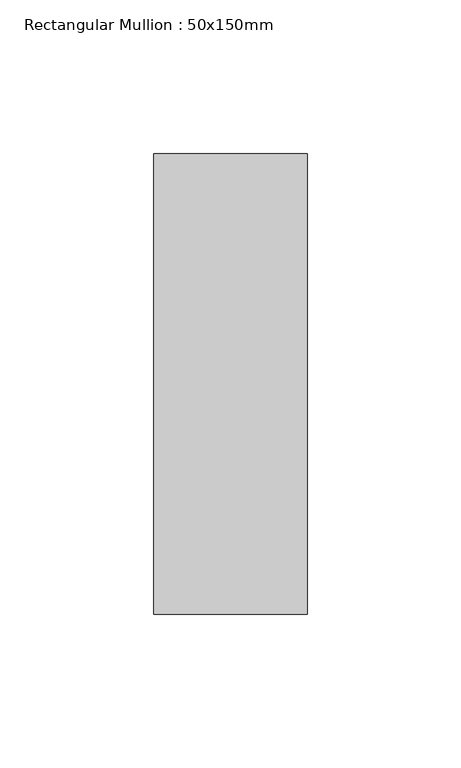
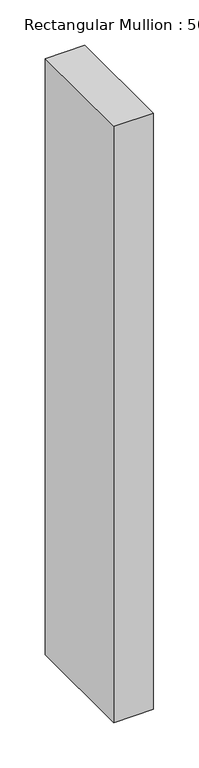
"""IFC4 building model written with IfcOpenShell, lengths in millimetres: member geometry, Rectangular Mullion : 50x150mm."""

from ifc_helpers import new_model, si_unit, frame, origin, place, context, project, spatial, polyline, outline, extrude, source, transform, mapped, element, save


def rectangular_mullion_50x150mm_14f10ac7(model_context):
    return source(origin(), model_context, "Body", "SweptSolid", [
        extrude(outline(polyline([(25.0, 75.0), (25.0, -75.0), (-25.0, -75.0), (-25.0, 75.0), (25.0, 75.0)])), frame((0.0, 0.0, -800.0), z_axis=(0.0, 0.0, 1.0), x_axis=(1.0, 0.0, 0.0)), (0.0, 0.0, 1.0), 800.0),
    ])


if __name__ == "__main__":
    model = new_model("IFC4")
    model_context = context("Model", 3, world=origin())
    ifc_project = project(units=[si_unit("LENGTHUNIT", "METRE", prefix="MILLI")], contexts=[model_context])
    site = spatial("IfcSite", under=ifc_project)
    building = spatial("IfcBuilding", under=site)
    placement = place(None, origin())
    rectangular_mullion_50x150mm_shape = rectangular_mullion_50x150mm_14f10ac7(model_context)
    element("IfcMember", 1, ObjectType="Rectangular Mullion : 50x150mm", at=placement, inside=building, context=model_context, shape_type="MappedRepresentation", body=[
        mapped(rectangular_mullion_50x150mm_shape, transform((0.0, 0.0, 0.0), x_axis=(1.0, 0.0, 0.0), y_axis=(0.0, 1.0, 0.0), z_axis=(0.0, 0.0, 1.0))),
    ])
    save(model, "model.ifc")

# Revit data of these elements
# Type "Rectangular Mullion : 50x150mm"
#   Keynote = "H11"
#   built-in parameter 1007304 = 0.492126 (stored number, unit not read)
#   built-in parameter 1007301 = 0.082021 (stored number, unit not read)
#   built-in parameter 1007300 = 0.082021 (stored number, unit not read)
# Element 1 (IfcMember, "Rectangular Mullion : 50x150mm")
#   Materials on its faces: "Aluminium"
# Materials
#   "Aluminium": class "Metal", colour RGB 247 247 247, transparency 0, Description = "Aluminium 6061", Cost = 0
